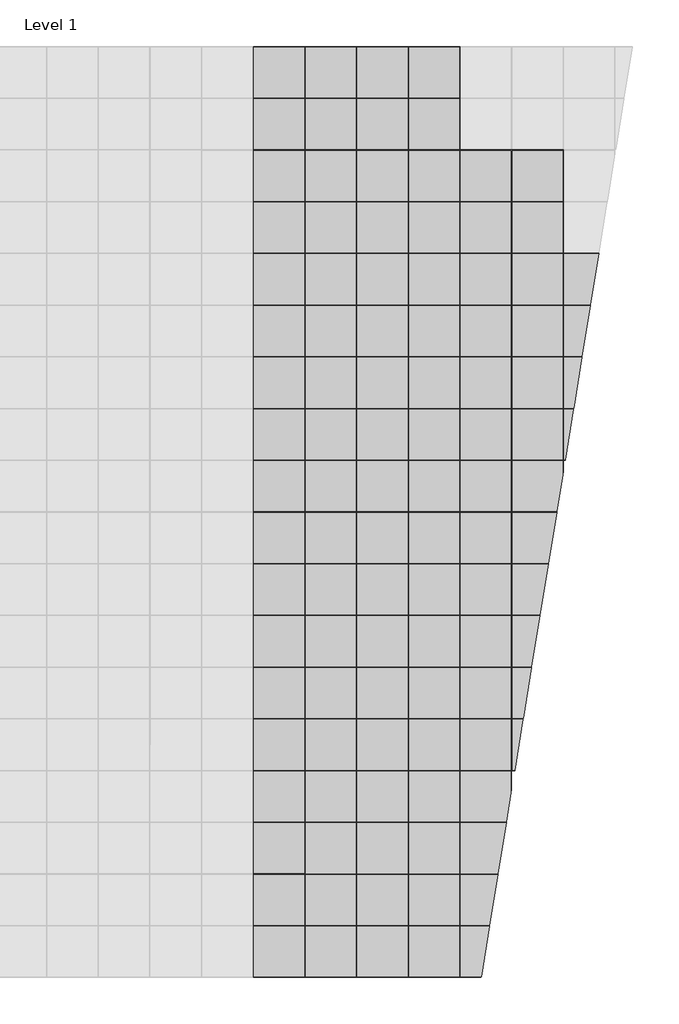
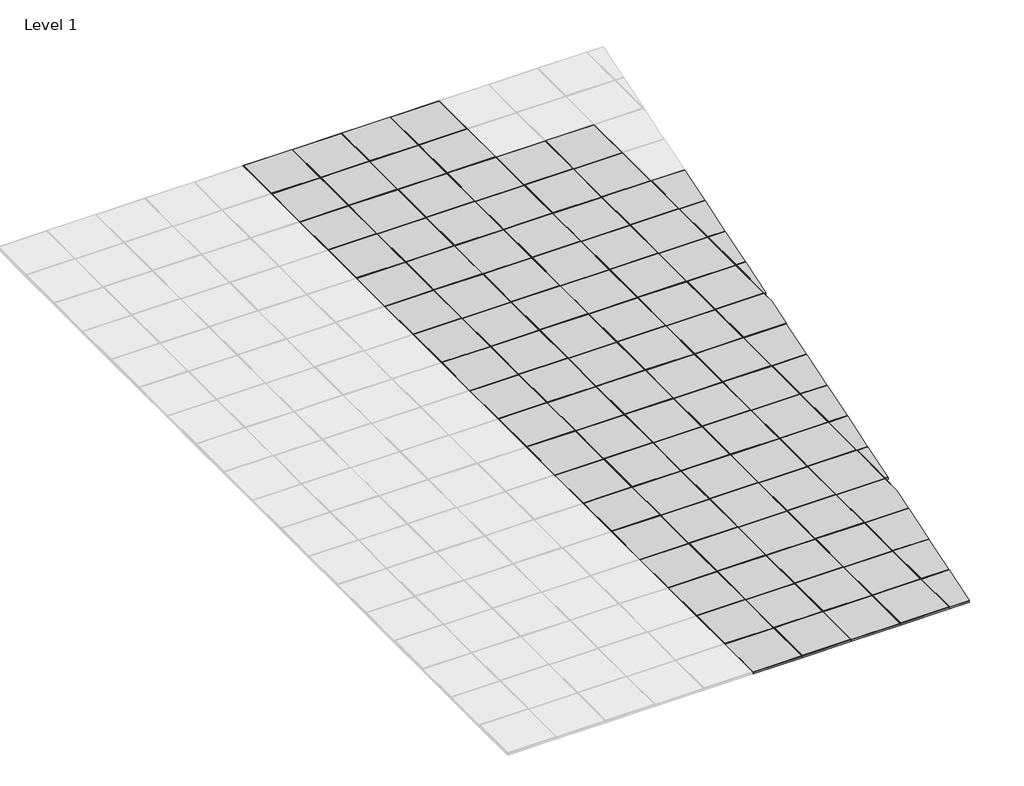
# One storey, part 2 of 18: 104 plates.
"""IFC4 building model written with IfcOpenShell, lengths in millimetres."""

import ifcopenshell
import ifcopenshell.guid

model = None  # the IFC model being written
_history = None  # IfcOwnerHistory: only IFC2X3 demands one
_inside = {}  # id of a spatial element -> (the spatial element, [elements in it])
_under = {}  # id of a project, library or spatial element -> (it, [spatial elements below it])
_declared = {}  # id of a project -> (the project, [libraries it declares])
_typed = {}  # id of a type object -> (the type object, [elements of that type])
_made_of = {}  # id of a material, layer set ... -> (it, [elements and type objects made of it])


def new_model(schema):
    """Start an empty IFC model of exactly this schema.

    Asked for "IFC4X3", IfcOpenShell would pick the latest addendum, in which some entities
    have other attributes; the version numbers below select the first issue.
    IFC2X3 requires an IfcOwnerHistory on every rooted entity: one is made here for all.
    """
    global model, _history
    if schema == "IFC4X3":
        model = ifcopenshell.file(schema_version=(4, 3, 0, 0))
    else:
        model = ifcopenshell.file(schema=schema)
    _inside.clear()
    _under.clear()
    _declared.clear()
    _typed.clear()
    _made_of.clear()
    _history = None
    if model.schema == "IFC2X3":
        org = make("IfcOrganization", Name="unknown")
        user = make(
            "IfcPersonAndOrganization",
            ThePerson=make("IfcPerson", FamilyName="unknown"),
            TheOrganization=org,
        )
        app = make(
            "IfcApplication",
            ApplicationDeveloper=org,
            Version="unknown",
            ApplicationFullName="unknown",
            ApplicationIdentifier="unknown",
        )
        _history = make(
            "IfcOwnerHistory",
            OwningUser=user,
            OwningApplication=app,
            ChangeAction="ADDED",
            CreationDate=0,
        )
    return model


def make(cls, **values):
    """One entity of the class cls with the attributes given. An attribute that is None is left unset."""
    return model.create_entity(
        cls, **{name: value for name, value in values.items() if value is not None}
    )


def rooted(cls, **values):
    """An entity with a GlobalId (a new one), such as an element, a storey or a relation."""
    return make(cls, GlobalId=ifcopenshell.guid.new(), OwnerHistory=_history, **values)


def si_unit(unit_type, name, prefix=None):
    """IfcSIUnit, for example si_unit("LENGTHUNIT", "METRE", prefix="MILLI")."""
    return make("IfcSIUnit", UnitType=unit_type, Prefix=prefix, Name=name)


def assignment(units):
    """IfcUnitAssignment: the units of a project."""
    return None if units is None else make("IfcUnitAssignment", Units=units)


def point(xyz):
    """IfcCartesianPoint."""
    return None if xyz is None else make("IfcCartesianPoint", Coordinates=xyz)


def direction(xyz):
    """IfcDirection."""
    return None if xyz is None else make("IfcDirection", DirectionRatios=xyz)


def frame(location, z_axis=None, x_axis=None):
    """IfcAxis2Placement3D, a coordinate frame: its origin and axes. An axis left out is left unset."""
    return make(
        "IfcAxis2Placement3D",
        Location=point(location),
        Axis=direction(z_axis),
        RefDirection=direction(x_axis),
    )


def origin():
    """The frame at (0, 0, 0) with its axes left unset."""
    return frame((0.0, 0.0, 0.0))


def origin_with_axes():
    """The frame at (0, 0, 0) with the z axis (0, 0, 1) and the x axis (1, 0, 0) written out."""
    return frame((0.0, 0.0, 0.0), z_axis=(0.0, 0.0, 1.0), x_axis=(1.0, 0.0, 0.0))


def place(relative_to, where):
    """IfcLocalPlacement: puts the frame where relative to a parent placement (None: the world)."""
    return make(
        "IfcLocalPlacement", PlacementRelTo=relative_to, RelativePlacement=where
    )


def context(
    kind, dimensions, precision=None, world=None, true_north=None, identifier=None
):
    """IfcGeometricRepresentationContext, for example the 3D "Model" context."""
    return make(
        "IfcGeometricRepresentationContext",
        ContextIdentifier=identifier,
        ContextType=kind,
        CoordinateSpaceDimension=dimensions,
        Precision=precision,
        WorldCoordinateSystem=world,
        TrueNorth=true_north,
    )


def project(units=None, contexts=None):
    """IfcProject with its units and contexts."""
    return rooted(
        "IfcProject",
        Name="project",
        RepresentationContexts=contexts,
        UnitsInContext=assignment(units),
    )


def spatial(cls, under=None, at=None, **own):
    """A site, building, storey or space (cls), placed at a placement, below another one or the project."""
    s = rooted(cls, ObjectPlacement=at, **own)
    if under is not None:
        _under.setdefault(under.id(), (under, []))[1].append(s)
    return s


def polyline(points):
    """IfcPolyline through the points."""
    return make("IfcPolyline", Points=[point(p) for p in points])


def outline(outer, holes=None, kind="AREA"):
    """IfcArbitraryClosedProfileDef: a profile drawn as a closed curve; with holes, ...WithVoids."""
    if holes is None:
        return make("IfcArbitraryClosedProfileDef", ProfileType=kind, OuterCurve=outer)
    return make(
        "IfcArbitraryProfileDefWithVoids",
        ProfileType=kind,
        OuterCurve=outer,
        InnerCurves=holes,
    )


def extrude(swept, where, along, depth):
    """IfcExtrudedAreaSolid: the profile swept, set in the frame where, extruded along a direction by depth."""
    return make(
        "IfcExtrudedAreaSolid",
        SweptArea=swept,
        Position=where,
        ExtrudedDirection=direction(along),
        Depth=depth,
    )


def shape(context_of_items, identifier, shape_type, items):
    """IfcShapeRepresentation: the items that make up one representation, for example the "Body"."""
    return make(
        "IfcShapeRepresentation",
        ContextOfItems=context_of_items,
        RepresentationIdentifier=identifier,
        RepresentationType=shape_type,
        Items=items,
    )


def source(mapping_origin, context_of_items, identifier, shape_type, items):
    """IfcRepresentationMap: a shape defined once, which mapped items show again and again."""
    return make(
        "IfcRepresentationMap",
        MappingOrigin=mapping_origin,
        MappedRepresentation=shape(context_of_items, identifier, shape_type, items),
    )


def transform(
    local_origin,
    x_axis=None,
    y_axis=None,
    z_axis=None,
    scale=None,
    scale2=None,
    scale3=None,
    uniform=True,
):
    """IfcCartesianTransformationOperator3D, or its non-uniform kind. x_axis, y_axis, z_axis: its Axis1, 2, 3."""
    if uniform:
        return make(
            "IfcCartesianTransformationOperator3D",
            Axis1=direction(x_axis),
            Axis2=direction(y_axis),
            LocalOrigin=point(local_origin),
            Scale=scale,
            Axis3=direction(z_axis),
        )
    return make(
        "IfcCartesianTransformationOperator3DnonUniform",
        Axis1=direction(x_axis),
        Axis2=direction(y_axis),
        LocalOrigin=point(local_origin),
        Scale=scale,
        Axis3=direction(z_axis),
        Scale2=scale2,
        Scale3=scale3,
    )


def mapped(mapping_source, mapping_target):
    """IfcMappedItem: shows the shape of a source again, moved by a transform."""
    return make(
        "IfcMappedItem", MappingSource=mapping_source, MappingTarget=mapping_target
    )


def made_of(thing, what):
    """Note that an element or type object is made of a material, layer set ...; save() writes the relation."""
    if what is not None:
        _made_of.setdefault(what.id(), (what, []))[1].append(thing)
    return thing


def element(
    cls,
    number,
    at=None,
    inside=None,
    cuts=None,
    type_object=None,
    material=None,
    context=None,
    identifier="Body",
    shape_type=None,
    held_by="IfcProductDefinitionShape",
    body=None,
    shapes=None,
    **own,
):
    """One element of the class cls, such as IfcWall. Its Tag is "e" and its number.

    at: its placement. inside: the storey or other place that contains it. cuts: it is an
    opening in that element (IfcRelVoidsElement). A single representation is given by context,
    identifier, shape_type and body (its items); several are given by shapes. held_by: the class
    of the entity that holds the representations. save() writes the other relations.
    """
    e = rooted(cls, Tag="e%d" % number, ObjectPlacement=at, **own)
    if body is not None:
        shapes = [shape(context, identifier, shape_type, body)]
    if shapes is not None:
        e.Representation = make(held_by, Representations=shapes)
    if inside is not None:
        _inside.setdefault(inside.id(), (inside, []))[1].append(e)
    if cuts is not None:
        rooted(
            "IfcRelVoidsElement", RelatingBuildingElement=cuts, RelatedOpeningElement=e
        )
    if type_object is not None:
        _typed.setdefault(type_object.id(), (type_object, []))[1].append(e)
    return made_of(e, material)


def aggregate(whole, parts):
    """IfcRelAggregates: a whole, such as a stair, and the parts it consists of."""
    return rooted("IfcRelAggregates", RelatingObject=whole, RelatedObjects=parts)


def save(model, path):
    """Write the relations noted so far, then the file.

    IfcRelAggregates (storeys below a building ...), IfcRelContainedInSpatialStructure (elements
    in a storey), IfcRelDefinesByType, IfcRelAssociatesMaterial and IfcRelDeclares: one each for
    every whole, place, type object, material and project.
    """
    for whole, parts in _under.values():
        aggregate(whole, parts)
    for where, things in _inside.values():
        rooted(
            "IfcRelContainedInSpatialStructure",
            RelatedElements=things,
            RelatingStructure=where,
        )
    for kind, things in _typed.values():
        rooted("IfcRelDefinesByType", RelatedObjects=things, RelatingType=kind)
    for what, things in _made_of.values():
        rooted("IfcRelAssociatesMaterial", RelatedObjects=things, RelatingMaterial=what)
    for by, libraries in _declared.values():
        rooted("IfcRelDeclares", RelatingContext=by, RelatedDefinitions=libraries)
    model.write(path)


def type_1_8eb2385c(model_context):
    return source(origin(), model_context, "Body", "SweptSolid", [
        extrude(outline(polyline([(1000.0, 500.0), (500.0, 500.0), (500.0, 1000.0), (1000.0, 1000.0), (1000.0, 500.0)]), holes=[polyline([(995.0, 995.0), (505.0, 995.0), (505.0, 505.0), (995.0, 505.0), (995.0, 995.0)])]), origin_with_axes(), (0.0, 0.0, 1.0), 18.0),
        extrude(outline(polyline([(505.0, 995.0), (995.0, 995.0), (995.0, 505.0), (505.0, 505.0), (505.0, 995.0)])), origin_with_axes(), (0.0, 0.0, 1.0), 20.0),
    ])


model = new_model("IFC4")

# Units and contexts
model_context = context("Model", 3, world=origin())
ifc_project = project(units=[si_unit("LENGTHUNIT", "METRE", prefix="MILLI")], contexts=[model_context])

# Site, building, storey
site = spatial("IfcSite", under=ifc_project)
building = spatial("IfcBuilding", under=site)
storey = spatial("IfcBuildingStorey", under=building, Name="Level 1", Elevation=0.0)

# Plates
placement = place(None, origin())
element("IfcPlate", 1, ObjectType="00_CPA_tegel : Type 1", at=placement, inside=storey, context=model_context, shape_type="SweptSolid", body=[
    extrude(outline(polyline([(2554.2097958, -16904.4539394), (2554.2195786, -16414.4539395), (2834.3103439, -16414.4595315), (2754.6354735, -16904.4579409), (2554.2097958, -16904.4539394)])), frame((0.0, 0.0, 1000.0), z_axis=(0.0, 0.0, 1.0), x_axis=(1.0, 0.0, 0.0)), (0.0, 0.0, 1.0), 20.0),
    extrude(outline(polyline([(2549.209696, -16909.4538396), (2549.2196784, -16409.4538397), (2835.1233527, -16409.4595477), (2834.3103439, -16414.4595315), (2554.2195786, -16414.4539395), (2554.2097958, -16904.4539394), (2754.6354735, -16904.4579409), (2753.8224647, -16909.4579246), (2549.209696, -16909.4538396)])), frame((0.0, 0.0, 1000.0), z_axis=(0.0, 0.0, 1.0), x_axis=(1.0, 0.0, 0.0)), (0.0, 0.0, 1.0), 18.0),
])
element("IfcPlate", 2, ObjectType="00_CPA_tegel : Type 1", at=placement, inside=storey, context=model_context, shape_type="SweptSolid", body=[
    extrude(outline(polyline([(2554.2197783, -16404.4539395), (2554.229561, -15914.4539396), (2915.6112321, -15914.4611545), (2835.9363617, -16404.4595639), (2554.2197783, -16404.4539395)])), frame((0.0, 0.0, 1000.0), z_axis=(0.0, 0.0, 1.0), x_axis=(1.0, 0.0, 0.0)), (0.0, 0.0, 1.0), 20.0),
    extrude(outline(polyline([(2549.2196784, -16409.4538397), (2549.2296609, -15909.4538398), (2916.424241, -15909.4611708), (2915.6112321, -15914.4611545), (2554.229561, -15914.4539396), (2554.2197783, -16404.4539395), (2835.9363617, -16404.4595639), (2835.1233528, -16409.4595477), (2549.2196784, -16409.4538397)])), frame((0.0, 0.0, 1000.0), z_axis=(0.0, 0.0, 1.0), x_axis=(1.0, 0.0, 0.0)), (0.0, 0.0, 1.0), 18.0),
])
element("IfcPlate", 3, ObjectType="00_CPA_tegel : Type 1", at=placement, inside=storey, context=model_context, shape_type="SweptSolid", body=[
    extrude(outline(polyline([(2554.2297607, -15904.4539396), (2554.2395435, -15414.4539397), (2996.9121201, -15414.4627776), (2917.2372499, -15904.461187), (2554.2297607, -15904.4539396)])), frame((0.0, 0.0, 1000.0), z_axis=(0.0, 0.0, 1.0), x_axis=(1.0, 0.0, 0.0)), (0.0, 0.0, 1.0), 20.0),
    extrude(outline(polyline([(2549.2296609, -15909.4538398), (2549.2396433, -15409.4538399), (2997.7251291, -15409.4627938), (2996.9121203, -15414.4627776), (2554.2395435, -15414.4539397), (2554.2297607, -15904.4539396), (2917.2372499, -15904.461187), (2916.424241, -15909.4611708), (2549.2296609, -15909.4538398)])), frame((0.0, 0.0, 1000.0), z_axis=(0.0, 0.0, 1.0), x_axis=(1.0, 0.0, 0.0)), (0.0, 0.0, 1.0), 18.0),
])
element("IfcPlate", 4, ObjectType="00_CPA_tegel : Type 1", at=placement, inside=storey, context=model_context, shape_type="SweptSolid", body=[
    extrude(outline(polyline([(2554.2397431, -15404.4539397), (2554.2495259, -14914.4539398), (3044.2495258, -14914.4637226), (3044.2453551, -15123.3645971), (2998.538138, -15404.4628101), (2554.2397431, -15404.4539397)])), frame((0.0, 0.0, 1000.0), z_axis=(0.0, 0.0, 1.0), x_axis=(1.0, 0.0, 0.0)), (0.0, 0.0, 1.0), 20.0),
    extrude(outline(polyline([(2549.2496257, -14909.45384), (3049.2496256, -14909.4638224), (3049.2459691, -15092.6109493), (3044.2453551, -15123.3645971), (3044.2495258, -14914.4637226), (2554.2495259, -14914.4539398), (2554.2397431, -15404.4539397), (2998.538138, -15404.4628101), (2997.7251291, -15409.4627938), (2549.2396433, -15409.4538399), (2549.2496257, -14909.45384)])), frame((0.0, 0.0, 1000.0), z_axis=(0.0, 0.0, 1.0), x_axis=(1.0, 0.0, 0.0)), (0.0, 0.0, 1.0), 18.0),
])
element("IfcPlate", 5, ObjectType="00_CPA_tegel : Type 1", at=placement, inside=storey, context=model_context, shape_type="SweptSolid", body=[
    extrude(outline(polyline([(2554.2497256, -14904.4539398), (2554.2595083, -14414.4539399), (3044.2595082, -14414.4637227), (3044.2497255, -14904.4637226), (2554.2497256, -14904.4539398)])), frame((0.0, 0.0, 1000.0), z_axis=(0.0, 0.0, 1.0), x_axis=(1.0, 0.0, 0.0)), (0.0, 0.0, 1.0), 20.0),
    extrude(outline(polyline([(3049.2496256, -14909.4638224), (2549.2496257, -14909.45384), (2549.2596082, -14409.4538401), (3049.2596081, -14409.4638225), (3049.2496256, -14909.4638224)]), holes=[polyline([(3044.2595082, -14414.4637227), (2554.2595083, -14414.4539399), (2554.2497256, -14904.4539398), (3044.2497255, -14904.4637226), (3044.2595082, -14414.4637227)])]), frame((0.0, 0.0, 1000.0), z_axis=(0.0, 0.0, 1.0), x_axis=(1.0, 0.0, 0.0)), (0.0, 0.0, 1.0), 18.0),
])
element("IfcPlate", 6, ObjectType="00_CPA_tegel : Type 1", at=placement, inside=storey, context=model_context, shape_type="SweptSolid", body=[
    extrude(outline(polyline([(3054.2497255, -14904.4639222), (3054.2595082, -14414.4639223), (3159.5138967, -14414.4660237), (3079.8390262, -14904.4644331), (3054.2497255, -14904.4639222)])), frame((0.0, 0.0, 1000.0), z_axis=(0.0, 0.0, 1.0), x_axis=(1.0, 0.0, 0.0)), (0.0, 0.0, 1.0), 20.0),
    extrude(outline(polyline([(3049.2496256, -14909.4638224), (3049.2596081, -14409.4638225), (3160.3269056, -14409.46604), (3159.5138966, -14414.4660237), (3054.2595082, -14414.4639223), (3054.2497255, -14904.4639222), (3079.8390262, -14904.4644331), (3079.0260173, -14909.4644169), (3049.2496256, -14909.4638224)])), frame((0.0, 0.0, 1000.0), z_axis=(0.0, 0.0, 1.0), x_axis=(1.0, 0.0, 0.0)), (0.0, 0.0, 1.0), 18.0),
])
element("IfcPlate", 7, ObjectType="00_CPA_tegel : Type 1", at=placement, inside=storey, context=model_context, shape_type="SweptSolid", body=[
    extrude(outline(polyline([(3554.3295848, -10904.4739055), (3554.3393676, -10414.4739056), (3809.9210017, -10414.4790082), (3730.2461314, -10904.4774176), (3554.3295848, -10904.4739055)])), frame((0.0, 0.0, 1000.0), z_axis=(0.0, 0.0, 1.0), x_axis=(1.0, 0.0, 0.0)), (0.0, 0.0, 1.0), 20.0),
    extrude(outline(polyline([(3549.329485, -10909.4738056), (3549.3394674, -10409.4738057), (3810.7340106, -10409.4790245), (3809.9210018, -10414.4790082), (3554.3393676, -10414.4739056), (3554.3295848, -10904.4739055), (3730.2461314, -10904.4774176), (3729.4331225, -10909.4774014), (3549.329485, -10909.4738056)])), frame((0.0, 0.0, 1000.0), z_axis=(0.0, 0.0, 1.0), x_axis=(1.0, 0.0, 0.0)), (0.0, 0.0, 1.0), 18.0),
])
element("IfcPlate", 8, ObjectType="00_CPA_tegel : Type 1", at=placement, inside=storey, context=model_context, shape_type="SweptSolid", body=[
    extrude(outline(polyline([(3554.3395673, -10404.4739056), (3554.34935, -9914.4739057), (3891.2218899, -9914.4806313), (3811.5470196, -10404.4790407), (3554.3395673, -10404.4739056)])), frame((0.0, 0.0, 1000.0), z_axis=(0.0, 0.0, 1.0), x_axis=(1.0, 0.0, 0.0)), (0.0, 0.0, 1.0), 20.0),
    extrude(outline(polyline([(3549.3394674, -10409.4738057), (3549.3494499, -9909.4738058), (3892.0348988, -9909.4806475), (3891.22189, -9914.4806313), (3554.34935, -9914.4739057), (3554.3395673, -10404.4739056), (3811.5470196, -10404.4790407), (3810.7340107, -10409.4790245), (3549.3394674, -10409.4738057)])), frame((0.0, 0.0, 1000.0), z_axis=(0.0, 0.0, 1.0), x_axis=(1.0, 0.0, 0.0)), (0.0, 0.0, 1.0), 18.0),
])
element("IfcPlate", 9, ObjectType="00_CPA_tegel : Type 1", at=placement, inside=storey, context=model_context, shape_type="SweptSolid", body=[
    extrude(outline(polyline([(3054.2597079, -14404.4639223), (3054.2694907, -13914.4639224), (3240.8147847, -13914.4676468), (3161.1399143, -14404.4660562), (3054.2597079, -14404.4639223)])), frame((0.0, 0.0, 1000.0), z_axis=(0.0, 0.0, 1.0), x_axis=(1.0, 0.0, 0.0)), (0.0, 0.0, 1.0), 20.0),
    extrude(outline(polyline([(3049.2596081, -14409.4638225), (3049.2695905, -13909.4638226), (3241.6277936, -13909.467663), (3240.8147847, -13914.4676468), (3054.2694907, -13914.4639224), (3054.2597079, -14404.4639223), (3161.1399143, -14404.4660562), (3160.3269054, -14409.46604), (3049.2596081, -14409.4638225)])), frame((0.0, 0.0, 1000.0), z_axis=(0.0, 0.0, 1.0), x_axis=(1.0, 0.0, 0.0)), (0.0, 0.0, 1.0), 18.0),
])
element("IfcPlate", 10, ObjectType="00_CPA_tegel : Type 1", at=placement, inside=storey, context=model_context, shape_type="SweptSolid", body=[
    extrude(outline(polyline([(3054.2696903, -13904.4639224), (3054.2794731, -13414.4639225), (3322.1156728, -13414.4692699), (3242.4408025, -13904.4676793), (3054.2696903, -13904.4639224)])), frame((0.0, 0.0, 1000.0), z_axis=(0.0, 0.0, 1.0), x_axis=(1.0, 0.0, 0.0)), (0.0, 0.0, 1.0), 20.0),
    extrude(outline(polyline([(3049.2695905, -13909.4638226), (3049.2795729, -13409.4638227), (3322.9286817, -13409.4692861), (3322.1156729, -13414.4692699), (3054.2794731, -13414.4639225), (3054.2696903, -13904.4639224), (3242.4408025, -13904.4676793), (3241.6277936, -13909.467663), (3049.2695905, -13909.4638226)])), frame((0.0, 0.0, 1000.0), z_axis=(0.0, 0.0, 1.0), x_axis=(1.0, 0.0, 0.0)), (0.0, 0.0, 1.0), 18.0),
])
element("IfcPlate", 11, ObjectType="00_CPA_tegel : Type 1", at=placement, inside=storey, context=model_context, shape_type="SweptSolid", body=[
    extrude(outline(polyline([(3054.2796728, -13404.4639225), (3054.2894555, -12914.4639226), (3403.416561, -12914.4708929), (3323.7416906, -13404.4693023), (3054.2796728, -13404.4639225)])), frame((0.0, 0.0, 1000.0), z_axis=(0.0, 0.0, 1.0), x_axis=(1.0, 0.0, 0.0)), (0.0, 0.0, 1.0), 20.0),
    extrude(outline(polyline([(3049.2795729, -13409.4638227), (3049.2895554, -12909.4638228), (3404.2295699, -12909.4709091), (3403.416561, -12914.4708929), (3054.2894555, -12914.4639226), (3054.2796728, -13404.4639225), (3323.7416906, -13404.4693023), (3322.9286818, -13409.4692861), (3049.2795729, -13409.4638227)])), frame((0.0, 0.0, 1000.0), z_axis=(0.0, 0.0, 1.0), x_axis=(1.0, 0.0, 0.0)), (0.0, 0.0, 1.0), 18.0),
])
element("IfcPlate", 12, ObjectType="00_CPA_tegel : Type 1", at=placement, inside=storey, context=model_context, shape_type="SweptSolid", body=[
    extrude(outline(polyline([(3054.2896552, -12904.4639226), (3054.299438, -12414.4639227), (3484.7174491, -12414.472516), (3405.0425788, -12904.4709254), (3054.2896552, -12904.4639226)])), frame((0.0, 0.0, 1000.0), z_axis=(0.0, 0.0, 1.0), x_axis=(1.0, 0.0, 0.0)), (0.0, 0.0, 1.0), 20.0),
    extrude(outline(polyline([(3049.2895554, -12909.4638228), (3049.2995378, -12409.4638229), (3485.5304581, -12409.4725322), (3484.7174492, -12414.472516), (3054.299438, -12414.4639227), (3054.2896552, -12904.4639226), (3405.0425788, -12904.4709254), (3404.2295699, -12909.4709091), (3049.2895554, -12909.4638228)])), frame((0.0, 0.0, 1000.0), z_axis=(0.0, 0.0, 1.0), x_axis=(1.0, 0.0, 0.0)), (0.0, 0.0, 1.0), 18.0),
])
element("IfcPlate", 13, ObjectType="00_CPA_tegel : Type 1", at=placement, inside=storey, context=model_context, shape_type="SweptSolid", body=[
    extrude(outline(polyline([(3054.2996376, -12404.4639227), (3054.3094204, -11914.4639228), (3544.3094203, -11914.4737056), (3544.3067545, -12047.9998168), (3486.343467, -12404.4725484), (3054.2996376, -12404.4639227)])), frame((0.0, 0.0, 1000.0), z_axis=(0.0, 0.0, 1.0), x_axis=(1.0, 0.0, 0.0)), (0.0, 0.0, 1.0), 20.0),
    extrude(outline(polyline([(3049.3095202, -11909.463823), (3549.3095201, -11909.4738054), (3549.3073685, -12017.246169), (3544.3067545, -12047.9998168), (3544.3094203, -11914.4737056), (3054.3094204, -11914.4639228), (3054.2996376, -12404.4639227), (3486.343467, -12404.4725484), (3485.5304581, -12409.4725322), (3049.2995378, -12409.4638229), (3049.3095202, -11909.463823)])), frame((0.0, 0.0, 1000.0), z_axis=(0.0, 0.0, 1.0), x_axis=(1.0, 0.0, 0.0)), (0.0, 0.0, 1.0), 18.0),
])
element("IfcPlate", 14, ObjectType="00_CPA_tegel : Type 1", at=placement, inside=storey, context=model_context, shape_type="SweptSolid", body=[
    extrude(outline(polyline([(3054.3096201, -11904.4639228), (3054.3194028, -11414.4639229), (3544.3194027, -11414.4737057), (3544.30962, -11904.4737056), (3054.3096201, -11904.4639228)])), frame((0.0, 0.0, 1000.0), z_axis=(0.0, 0.0, 1.0), x_axis=(1.0, 0.0, 0.0)), (0.0, 0.0, 1.0), 20.0),
    extrude(outline(polyline([(3549.3095201, -11909.4738054), (3049.3095202, -11909.463823), (3049.3195027, -11409.4638231), (3549.3195026, -11409.4738055), (3549.3095201, -11909.4738054)]), holes=[polyline([(3544.3194027, -11414.4737057), (3054.3194028, -11414.4639229), (3054.3096201, -11904.4639228), (3544.30962, -11904.4737056), (3544.3194027, -11414.4737057)])]), frame((0.0, 0.0, 1000.0), z_axis=(0.0, 0.0, 1.0), x_axis=(1.0, 0.0, 0.0)), (0.0, 0.0, 1.0), 18.0),
])
element("IfcPlate", 15, ObjectType="00_CPA_tegel : Type 1", at=placement, inside=storey, context=model_context, shape_type="SweptSolid", body=[
    extrude(outline(polyline([(3554.30962, -11904.4739053), (3554.3194027, -11414.4739054), (3647.3192254, -11414.4757621), (3567.6443551, -11904.4741715), (3554.30962, -11904.4739053)])), frame((0.0, 0.0, 1000.0), z_axis=(0.0, 0.0, 1.0), x_axis=(1.0, 0.0, 0.0)), (0.0, 0.0, 1.0), 20.0),
    extrude(outline(polyline([(3549.3095201, -11909.4738054), (3549.3195026, -11409.4738055), (3648.1322344, -11409.4757783), (3647.3192255, -11414.4757621), (3554.3194027, -11414.4739054), (3554.30962, -11904.4739053), (3567.6443551, -11904.4741715), (3566.8313462, -11909.4741553), (3549.3095201, -11909.4738054)])), frame((0.0, 0.0, 1000.0), z_axis=(0.0, 0.0, 1.0), x_axis=(1.0, 0.0, 0.0)), (0.0, 0.0, 1.0), 18.0),
])
element("IfcPlate", 16, ObjectType="00_CPA_tegel : Type 1", at=placement, inside=storey, context=model_context, shape_type="SweptSolid", body=[
    extrude(outline(polyline([(3554.3196024, -11404.4739054), (3554.3293852, -10914.4739055), (3728.6201137, -10914.4773852), (3648.9452433, -11404.4757946), (3554.3196024, -11404.4739054)])), frame((0.0, 0.0, 1000.0), z_axis=(0.0, 0.0, 1.0), x_axis=(1.0, 0.0, 0.0)), (0.0, 0.0, 1.0), 20.0),
    extrude(outline(polyline([(3549.3195026, -11409.4738055), (3549.329485, -10909.4738056), (3729.4331225, -10909.4774014), (3728.6201137, -10914.4773852), (3554.3293852, -10914.4739055), (3554.3196024, -11404.4739054), (3648.9452433, -11404.4757946), (3648.1322344, -11409.4757783), (3549.3195026, -11409.4738055)])), frame((0.0, 0.0, 1000.0), z_axis=(0.0, 0.0, 1.0), x_axis=(1.0, 0.0, 0.0)), (0.0, 0.0, 1.0), 18.0),
])
type_1_shape = type_1_8eb2385c(model_context)
element("IfcPlate", 17, ObjectType="00_CPA_tegel : Type 1", at=placement, inside=storey, context=model_context, shape_type="MappedRepresentation", body=[
    mapped(type_1_shape, transform((49.1997141, -17409.4039273, 1000.0), x_axis=(0.9999999998007024, -1.9964866676991377e-05, 0.0), y_axis=(1.9964866676991377e-05, 0.9999999998007024, 0.0), z_axis=(0.0, 0.0, 1.0))),
])
element("IfcPlate", 18, ObjectType="00_CPA_tegel : Type 1", at=placement, inside=storey, context=model_context, shape_type="MappedRepresentation", body=[
    mapped(type_1_shape, transform((549.199714, -17409.4139098, 1000.0), x_axis=(0.9999999998007022, -1.9964866676547288e-05, 0.0), y_axis=(1.9964866676547288e-05, 0.9999999998007022, 0.0), z_axis=(0.0, 0.0, 1.0))),
])
element("IfcPlate", 19, ObjectType="00_CPA_tegel : Type 1", at=placement, inside=storey, context=model_context, shape_type="MappedRepresentation", body=[
    mapped(type_1_shape, transform((49.2096965, -16909.4039274, 1000.0), x_axis=(0.9999999998007024, -1.9964866676325244e-05, 0.0), y_axis=(1.9964866676325244e-05, 0.9999999998007024, 0.0), z_axis=(0.0, 0.0, 1.0))),
])
element("IfcPlate", 20, ObjectType="00_CPA_tegel : Type 1", at=placement, inside=storey, context=model_context, shape_type="MappedRepresentation", body=[
    mapped(type_1_shape, transform((549.2096964, -16909.4139098, 1000.0), x_axis=(0.9999999998007023, -1.9964866675492576e-05, 0.0), y_axis=(1.9964866675492576e-05, 0.9999999998007023, 0.0), z_axis=(0.0, 0.0, 1.0))),
])
element("IfcPlate", 21, ObjectType="00_CPA_tegel : Type 1", at=placement, inside=storey, context=model_context, shape_type="MappedRepresentation", body=[
    mapped(type_1_shape, transform((49.2196789, -16409.4039275, 1000.0), x_axis=(0.9999999998007023, -1.9964866675492576e-05, 0.0), y_axis=(1.9964866675492576e-05, 0.9999999998007023, 0.0), z_axis=(0.0, 0.0, 1.0))),
])
element("IfcPlate", 22, ObjectType="00_CPA_tegel : Type 1", at=placement, inside=storey, context=model_context, shape_type="MappedRepresentation", body=[
    mapped(type_1_shape, transform((549.2196788, -16409.4139099, 1000.0), x_axis=(0.9999999998007023, -1.9964866675492576e-05, 0.0), y_axis=(1.9964866675492576e-05, 0.9999999998007023, 0.0), z_axis=(0.0, 0.0, 1.0))),
])
element("IfcPlate", 23, ObjectType="00_CPA_tegel : Type 1", at=placement, inside=storey, context=model_context, shape_type="MappedRepresentation", body=[
    mapped(type_1_shape, transform((49.2296614, -15909.4039276, 1000.0), x_axis=(0.9999999998007024, -1.9964866676991377e-05, 0.0), y_axis=(1.9964866676991377e-05, 0.9999999998007024, 0.0), z_axis=(0.0, 0.0, 1.0))),
])
element("IfcPlate", 24, ObjectType="00_CPA_tegel : Type 1", at=placement, inside=storey, context=model_context, shape_type="MappedRepresentation", body=[
    mapped(type_1_shape, transform((549.2296613, -15909.41391, 1000.0), x_axis=(0.9999999998007024, -1.9964866676991377e-05, 0.0), y_axis=(1.9964866676991377e-05, 0.9999999998007024, 0.0), z_axis=(0.0, 0.0, 1.0))),
])
element("IfcPlate", 25, ObjectType="00_CPA_tegel : Type 1", at=placement, inside=storey, context=model_context, shape_type="MappedRepresentation", body=[
    mapped(type_1_shape, transform((49.2396438, -15409.4039277, 1000.0), x_axis=(0.9999999998007023, -1.9964866675492576e-05, 0.0), y_axis=(1.9964866675492576e-05, 0.9999999998007023, 0.0), z_axis=(0.0, 0.0, 1.0))),
])
element("IfcPlate", 26, ObjectType="00_CPA_tegel : Type 1", at=placement, inside=storey, context=model_context, shape_type="MappedRepresentation", body=[
    mapped(type_1_shape, transform((549.2396437, -15409.4139101, 1000.0), x_axis=(0.9999999998007024, -1.9964866676991377e-05, 0.0), y_axis=(1.9964866676991377e-05, 0.9999999998007024, 0.0), z_axis=(0.0, 0.0, 1.0))),
])
element("IfcPlate", 27, ObjectType="00_CPA_tegel : Type 1", at=placement, inside=storey, context=model_context, shape_type="MappedRepresentation", body=[
    mapped(type_1_shape, transform((49.2496262, -14909.4039278, 1000.0), x_axis=(0.9999999998007024, -1.9964866676991377e-05, 0.0), y_axis=(1.9964866676991377e-05, 0.9999999998007024, 0.0), z_axis=(0.0, 0.0, 1.0))),
])
element("IfcPlate", 28, ObjectType="00_CPA_tegel : Type 1", at=placement, inside=storey, context=model_context, shape_type="MappedRepresentation", body=[
    mapped(type_1_shape, transform((549.2496261, -14909.4139102, 1000.0), x_axis=(0.9999999998007024, -1.9964866676991377e-05, 0.0), y_axis=(1.9964866676991377e-05, 0.9999999998007024, 0.0), z_axis=(0.0, 0.0, 1.0))),
])
element("IfcPlate", 29, ObjectType="00_CPA_tegel : Type 1", at=placement, inside=storey, context=model_context, shape_type="MappedRepresentation", body=[
    mapped(type_1_shape, transform((49.2596087, -14409.4039279, 1000.0), x_axis=(0.9999999998007024, -1.9964866676991377e-05, 0.0), y_axis=(1.9964866676991377e-05, 0.9999999998007024, 0.0), z_axis=(0.0, 0.0, 1.0))),
])
element("IfcPlate", 30, ObjectType="00_CPA_tegel : Type 1", at=placement, inside=storey, context=model_context, shape_type="MappedRepresentation", body=[
    mapped(type_1_shape, transform((549.2596086, -14409.4139103, 1000.0), x_axis=(0.9999999998007024, -1.9964866676991377e-05, 0.0), y_axis=(1.9964866676991377e-05, 0.9999999998007024, 0.0), z_axis=(0.0, 0.0, 1.0))),
])
element("IfcPlate", 31, ObjectType="00_CPA_tegel : Type 1", at=placement, inside=storey, context=model_context, shape_type="MappedRepresentation", body=[
    mapped(type_1_shape, transform((49.2695911, -13909.403928, 1000.0), x_axis=(0.9999999998007022, -1.9964866678323645e-05, 0.0), y_axis=(1.9964866678323645e-05, 0.9999999998007022, 0.0), z_axis=(0.0, 0.0, 1.0))),
])
element("IfcPlate", 32, ObjectType="00_CPA_tegel : Type 1", at=placement, inside=storey, context=model_context, shape_type="MappedRepresentation", body=[
    mapped(type_1_shape, transform((549.269591, -13909.4139104, 1000.0), x_axis=(0.9999999998007024, -1.9964866676991377e-05, 0.0), y_axis=(1.9964866676991377e-05, 0.9999999998007024, 0.0), z_axis=(0.0, 0.0, 1.0))),
])
element("IfcPlate", 33, ObjectType="00_CPA_tegel : Type 1", at=placement, inside=storey, context=model_context, shape_type="MappedRepresentation", body=[
    mapped(type_1_shape, transform((49.2795735, -13409.4039281, 1000.0), x_axis=(0.9999999998007022, -1.9964866678323645e-05, 0.0), y_axis=(1.9964866678323645e-05, 0.9999999998007022, 0.0), z_axis=(0.0, 0.0, 1.0))),
])
element("IfcPlate", 34, ObjectType="00_CPA_tegel : Type 1", at=placement, inside=storey, context=model_context, shape_type="MappedRepresentation", body=[
    mapped(type_1_shape, transform((549.2795734, -13409.4139105, 1000.0), x_axis=(0.9999999998007024, -1.9964866676991377e-05, 0.0), y_axis=(1.9964866676991377e-05, 0.9999999998007024, 0.0), z_axis=(0.0, 0.0, 1.0))),
])
element("IfcPlate", 35, ObjectType="00_CPA_tegel : Type 1", at=placement, inside=storey, context=model_context, shape_type="MappedRepresentation", body=[
    mapped(type_1_shape, transform((1049.1997139, -17409.4238922, 1000.0), x_axis=(0.9999999998007023, -1.996486667804609e-05, 0.0), y_axis=(1.996486667804609e-05, 0.9999999998007023, 0.0), z_axis=(0.0, 0.0, 1.0))),
])
element("IfcPlate", 36, ObjectType="00_CPA_tegel : Type 1", at=placement, inside=storey, context=model_context, shape_type="MappedRepresentation", body=[
    mapped(type_1_shape, transform((1049.2096963, -16909.4238923, 1000.0), x_axis=(0.9999999998007024, -1.9964866676991377e-05, 0.0), y_axis=(1.9964866676991377e-05, 0.9999999998007024, 0.0), z_axis=(0.0, 0.0, 1.0))),
])
element("IfcPlate", 37, ObjectType="00_CPA_tegel : Type 1", at=placement, inside=storey, context=model_context, shape_type="MappedRepresentation", body=[
    mapped(type_1_shape, transform((1049.2196787, -16409.4238924, 1000.0), x_axis=(0.9999999998007022, -1.9964866678323645e-05, 0.0), y_axis=(1.9964866678323645e-05, 0.9999999998007022, 0.0), z_axis=(0.0, 0.0, 1.0))),
])
element("IfcPlate", 38, ObjectType="00_CPA_tegel : Type 1", at=placement, inside=storey, context=model_context, shape_type="MappedRepresentation", body=[
    mapped(type_1_shape, transform((1549.2096962, -16909.4338747, 1000.0), x_axis=(0.9999999998007024, -1.9964866676325244e-05, 0.0), y_axis=(1.9964866676325244e-05, 0.9999999998007024, 0.0), z_axis=(0.0, 0.0, 1.0))),
])
element("IfcPlate", 39, ObjectType="00_CPA_tegel : Type 1", at=placement, inside=storey, context=model_context, shape_type="MappedRepresentation", body=[
    mapped(type_1_shape, transform((1549.2196786, -16409.4338748, 1000.0), x_axis=(0.9999999998007024, -1.9964866676991377e-05, 0.0), y_axis=(1.9964866676991377e-05, 0.9999999998007024, 0.0), z_axis=(0.0, 0.0, 1.0))),
])
element("IfcPlate", 40, ObjectType="00_CPA_tegel : Type 1", at=placement, inside=storey, context=model_context, shape_type="MappedRepresentation", body=[
    mapped(type_1_shape, transform((1049.2296612, -15909.4238925, 1000.0), x_axis=(0.9999999998007022, -1.9964866678323645e-05, 0.0), y_axis=(1.9964866678323645e-05, 0.9999999998007022, 0.0), z_axis=(0.0, 0.0, 1.0))),
])
element("IfcPlate", 41, ObjectType="00_CPA_tegel : Type 1", at=placement, inside=storey, context=model_context, shape_type="MappedRepresentation", body=[
    mapped(type_1_shape, transform((1549.2296611, -15909.4338749, 1000.0), x_axis=(0.9999999998007024, -1.9964866676991377e-05, 0.0), y_axis=(1.9964866676991377e-05, 0.9999999998007024, 0.0), z_axis=(0.0, 0.0, 1.0))),
])
element("IfcPlate", 42, ObjectType="00_CPA_tegel : Type 1", at=placement, inside=storey, context=model_context, shape_type="MappedRepresentation", body=[
    mapped(type_1_shape, transform((1049.2396436, -15409.4238926, 1000.0), x_axis=(0.9999999998007024, -1.9964866676991377e-05, 0.0), y_axis=(1.9964866676991377e-05, 0.9999999998007024, 0.0), z_axis=(0.0, 0.0, 1.0))),
])
element("IfcPlate", 43, ObjectType="00_CPA_tegel : Type 1", at=placement, inside=storey, context=model_context, shape_type="MappedRepresentation", body=[
    mapped(type_1_shape, transform((1049.249626, -14909.4238927, 1000.0), x_axis=(0.9999999998007023, -1.9964866675492576e-05, 0.0), y_axis=(1.9964866675492576e-05, 0.9999999998007023, 0.0), z_axis=(0.0, 0.0, 1.0))),
])
element("IfcPlate", 44, ObjectType="00_CPA_tegel : Type 1", at=placement, inside=storey, context=model_context, shape_type="MappedRepresentation", body=[
    mapped(type_1_shape, transform((1049.2596085, -14409.4238928, 1000.0), x_axis=(0.9999999998007022, -1.9964866678323645e-05, 0.0), y_axis=(1.9964866678323645e-05, 0.9999999998007022, 0.0), z_axis=(0.0, 0.0, 1.0))),
])
element("IfcPlate", 45, ObjectType="00_CPA_tegel : Type 1", at=placement, inside=storey, context=model_context, shape_type="MappedRepresentation", body=[
    mapped(type_1_shape, transform((1049.2695909, -13909.4238929, 1000.0), x_axis=(0.9999999998007022, -1.9964866678323645e-05, 0.0), y_axis=(1.9964866678323645e-05, 0.9999999998007022, 0.0), z_axis=(0.0, 0.0, 1.0))),
])
element("IfcPlate", 46, ObjectType="00_CPA_tegel : Type 1", at=placement, inside=storey, context=model_context, shape_type="MappedRepresentation", body=[
    mapped(type_1_shape, transform((1049.2795733, -13409.423893, 1000.0), x_axis=(0.9999999998007024, -1.9964866676991377e-05, 0.0), y_axis=(1.9964866676991377e-05, 0.9999999998007024, 0.0), z_axis=(0.0, 0.0, 1.0))),
])
element("IfcPlate", 47, ObjectType="00_CPA_tegel : Type 1", at=placement, inside=storey, context=model_context, shape_type="MappedRepresentation", body=[
    mapped(type_1_shape, transform((1549.2396435, -15409.433875, 1000.0), x_axis=(0.9999999998007024, -1.9964866676991377e-05, 0.0), y_axis=(1.9964866676991377e-05, 0.9999999998007024, 0.0), z_axis=(0.0, 0.0, 1.0))),
])
element("IfcPlate", 48, ObjectType="00_CPA_tegel : Type 1", at=placement, inside=storey, context=model_context, shape_type="MappedRepresentation", body=[
    mapped(type_1_shape, transform((1549.2496259, -14909.4338751, 1000.0), x_axis=(0.9999999998007022, -1.9964866678323645e-05, 0.0), y_axis=(1.9964866678323645e-05, 0.9999999998007022, 0.0), z_axis=(0.0, 0.0, 1.0))),
])
element("IfcPlate", 49, ObjectType="00_CPA_tegel : Type 1", at=placement, inside=storey, context=model_context, shape_type="MappedRepresentation", body=[
    mapped(type_1_shape, transform((1549.2596084, -14409.4338752, 1000.0), x_axis=(0.9999999998007024, -1.9964866676991377e-05, 0.0), y_axis=(1.9964866676991377e-05, 0.9999999998007024, 0.0), z_axis=(0.0, 0.0, 1.0))),
])
element("IfcPlate", 50, ObjectType="00_CPA_tegel : Type 1", at=placement, inside=storey, context=model_context, shape_type="MappedRepresentation", body=[
    mapped(type_1_shape, transform((1549.2695908, -13909.4338753, 1000.0), x_axis=(0.9999999998007024, -1.9964866676991377e-05, 0.0), y_axis=(1.9964866676991377e-05, 0.9999999998007024, 0.0), z_axis=(0.0, 0.0, 1.0))),
])
element("IfcPlate", 51, ObjectType="00_CPA_tegel : Type 1", at=placement, inside=storey, context=model_context, shape_type="MappedRepresentation", body=[
    mapped(type_1_shape, transform((1549.2795732, -13409.4338754, 1000.0), x_axis=(0.9999999998007022, -1.9964866678323645e-05, 0.0), y_axis=(1.9964866678323645e-05, 0.9999999998007022, 0.0), z_axis=(0.0, 0.0, 1.0))),
])
element("IfcPlate", 52, ObjectType="00_CPA_tegel : Type 1", at=placement, inside=storey, context=model_context, shape_type="MappedRepresentation", body=[
    mapped(type_1_shape, transform((49.289556, -12909.4039282, 1000.0), x_axis=(0.9999999998007023, -1.9964866675492576e-05, 0.0), y_axis=(1.9964866675492576e-05, 0.9999999998007023, 0.0), z_axis=(0.0, 0.0, 1.0))),
])
element("IfcPlate", 53, ObjectType="00_CPA_tegel : Type 1", at=placement, inside=storey, context=model_context, shape_type="MappedRepresentation", body=[
    mapped(type_1_shape, transform((549.2895559, -12909.4139106, 1000.0), x_axis=(0.9999999998007023, -1.9964866675492576e-05, 0.0), y_axis=(1.9964866675492576e-05, 0.9999999998007023, 0.0), z_axis=(0.0, 0.0, 1.0))),
])
element("IfcPlate", 54, ObjectType="00_CPA_tegel : Type 1", at=placement, inside=storey, context=model_context, shape_type="MappedRepresentation", body=[
    mapped(type_1_shape, transform((1049.2895558, -12909.4238931, 1000.0), x_axis=(0.9999999998007023, -1.9964866675492576e-05, 0.0), y_axis=(1.9964866675492576e-05, 0.9999999998007023, 0.0), z_axis=(0.0, 0.0, 1.0))),
])
element("IfcPlate", 55, ObjectType="00_CPA_tegel : Type 1", at=placement, inside=storey, context=model_context, shape_type="MappedRepresentation", body=[
    mapped(type_1_shape, transform((1549.2895557, -12909.4338755, 1000.0), x_axis=(0.9999999998007022, -1.9964866678323645e-05, 0.0), y_axis=(1.9964866678323645e-05, 0.9999999998007022, 0.0), z_axis=(0.0, 0.0, 1.0))),
])
element("IfcPlate", 56, ObjectType="00_CPA_tegel : Type 1", at=placement, inside=storey, context=model_context, shape_type="MappedRepresentation", body=[
    mapped(type_1_shape, transform((1549.2995381, -12409.4338756, 1000.0), x_axis=(0.9999999998007023, -1.9964866675492576e-05, 0.0), y_axis=(1.9964866675492576e-05, 0.9999999998007023, 0.0), z_axis=(0.0, 0.0, 1.0))),
])
element("IfcPlate", 57, ObjectType="00_CPA_tegel : Type 1", at=placement, inside=storey, context=model_context, shape_type="MappedRepresentation", body=[
    mapped(type_1_shape, transform((549.2995383, -12409.4139107, 1000.0), x_axis=(0.9999999998007022, -1.9964866678323645e-05, 0.0), y_axis=(1.9964866678323645e-05, 0.9999999998007022, 0.0), z_axis=(0.0, 0.0, 1.0))),
])
element("IfcPlate", 58, ObjectType="00_CPA_tegel : Type 1", at=placement, inside=storey, context=model_context, shape_type="MappedRepresentation", body=[
    mapped(type_1_shape, transform((1049.2995382, -12409.4238932, 1000.0), x_axis=(0.9999999998007022, -1.9964866678323645e-05, 0.0), y_axis=(1.9964866678323645e-05, 0.9999999998007022, 0.0), z_axis=(0.0, 0.0, 1.0))),
])
element("IfcPlate", 59, ObjectType="00_CPA_tegel : Type 1", at=placement, inside=storey, context=model_context, shape_type="MappedRepresentation", body=[
    mapped(type_1_shape, transform((1549.1997138, -17409.4338746, 1000.0), x_axis=(0.9999999998007024, -1.9964866676991377e-05, 0.0), y_axis=(1.9964866676991377e-05, 0.9999999998007024, 0.0), z_axis=(0.0, 0.0, 1.0))),
])
element("IfcPlate", 60, ObjectType="00_CPA_tegel : Type 1", at=placement, inside=storey, context=model_context, shape_type="MappedRepresentation", body=[
    mapped(type_1_shape, transform((49.2995384, -12409.4039283, 1000.0), x_axis=(0.9999999998007023, -1.9964866675492576e-05, 0.0), y_axis=(1.9964866675492576e-05, 0.9999999998007023, 0.0), z_axis=(0.0, 0.0, 1.0))),
])
element("IfcPlate", 61, ObjectType="00_CPA_tegel : Type 1", at=placement, inside=storey, context=model_context, shape_type="MappedRepresentation", body=[
    mapped(type_1_shape, transform((1049.3095206, -11909.4238933, 1000.0), x_axis=(0.9999999998007024, -1.9964866676991377e-05, 0.0), y_axis=(1.9964866676991377e-05, 0.9999999998007024, 0.0), z_axis=(0.0, 0.0, 1.0))),
])
element("IfcPlate", 62, ObjectType="00_CPA_tegel : Type 1", at=placement, inside=storey, context=model_context, shape_type="MappedRepresentation", body=[
    mapped(type_1_shape, transform((1549.3095205, -11909.4338757, 1000.0), x_axis=(0.9999999998007022, -1.9964866678323645e-05, 0.0), y_axis=(1.9964866678323645e-05, 0.9999999998007022, 0.0), z_axis=(0.0, 0.0, 1.0))),
])
element("IfcPlate", 63, ObjectType="00_CPA_tegel : Type 1", at=placement, inside=storey, context=model_context, shape_type="MappedRepresentation", body=[
    mapped(type_1_shape, transform((49.3195033, -11409.4039285, 1000.0), x_axis=(0.9999999998007023, -1.9964866675492576e-05, 0.0), y_axis=(1.9964866675492576e-05, 0.9999999998007023, 0.0), z_axis=(0.0, 0.0, 1.0))),
])
element("IfcPlate", 64, ObjectType="00_CPA_tegel : Type 1", at=placement, inside=storey, context=model_context, shape_type="MappedRepresentation", body=[
    mapped(type_1_shape, transform((2049.3294853, -10909.4438583, 1000.0), x_axis=(0.9999999998007022, -1.9964866678323645e-05, 0.0), y_axis=(1.9964866678323645e-05, 0.9999999998007022, 0.0), z_axis=(0.0, 0.0, 1.0))),
])
element("IfcPlate", 65, ObjectType="00_CPA_tegel : Type 1", at=placement, inside=storey, context=model_context, shape_type="MappedRepresentation", body=[
    mapped(type_1_shape, transform((2549.3294852, -10909.4538408, 1000.0), x_axis=(0.9999999998007022, -1.9964866679711424e-05, 0.0), y_axis=(1.9964866679711424e-05, 0.9999999998007022, 0.0), z_axis=(0.0, 0.0, 1.0))),
])
element("IfcPlate", 66, ObjectType="00_CPA_tegel : Type 1", at=placement, inside=storey, context=model_context, shape_type="MappedRepresentation", body=[
    mapped(type_1_shape, transform((1549.3294854, -10909.4338759, 1000.0), x_axis=(0.9999999998007022, -1.9964866678323645e-05, 0.0), y_axis=(1.9964866678323645e-05, 0.9999999998007022, 0.0), z_axis=(0.0, 0.0, 1.0))),
])
element("IfcPlate", 67, ObjectType="00_CPA_tegel : Type 1", at=placement, inside=storey, context=model_context, shape_type="MappedRepresentation", body=[
    mapped(type_1_shape, transform((2049.2496258, -14909.4438575, 1000.0), x_axis=(0.9999999998007024, -1.9964866676991377e-05, 0.0), y_axis=(1.9964866676991377e-05, 0.9999999998007024, 0.0), z_axis=(0.0, 0.0, 1.0))),
])
element("IfcPlate", 68, ObjectType="00_CPA_tegel : Type 1", at=placement, inside=storey, context=model_context, shape_type="MappedRepresentation", body=[
    mapped(type_1_shape, transform((2049.2596083, -14409.4438576, 1000.0), x_axis=(0.9999999998007024, -1.9964866676991377e-05, 0.0), y_axis=(1.9964866676991377e-05, 0.9999999998007024, 0.0), z_axis=(0.0, 0.0, 1.0))),
])
element("IfcPlate", 69, ObjectType="00_CPA_tegel : Type 1", at=placement, inside=storey, context=model_context, shape_type="MappedRepresentation", body=[
    mapped(type_1_shape, transform((2049.2695907, -13909.4438577, 1000.0), x_axis=(0.9999999998007022, -1.9964866678323645e-05, 0.0), y_axis=(1.9964866678323645e-05, 0.9999999998007022, 0.0), z_axis=(0.0, 0.0, 1.0))),
])
element("IfcPlate", 70, ObjectType="00_CPA_tegel : Type 1", at=placement, inside=storey, context=model_context, shape_type="MappedRepresentation", body=[
    mapped(type_1_shape, transform((2049.2795731, -13409.4438578, 1000.0), x_axis=(0.9999999998007024, -1.9964866676991377e-05, 0.0), y_axis=(1.9964866676991377e-05, 0.9999999998007024, 0.0), z_axis=(0.0, 0.0, 1.0))),
])
element("IfcPlate", 71, ObjectType="00_CPA_tegel : Type 1", at=placement, inside=storey, context=model_context, shape_type="MappedRepresentation", body=[
    mapped(type_1_shape, transform((2049.2895556, -12909.4438579, 1000.0), x_axis=(0.9999999998007024, -1.9964866676991377e-05, 0.0), y_axis=(1.9964866676991377e-05, 0.9999999998007024, 0.0), z_axis=(0.0, 0.0, 1.0))),
])
element("IfcPlate", 72, ObjectType="00_CPA_tegel : Type 1", at=placement, inside=storey, context=model_context, shape_type="MappedRepresentation", body=[
    mapped(type_1_shape, transform((2049.299538, -12409.443858, 1000.0), x_axis=(0.9999999998007024, -1.9964866676991377e-05, 0.0), y_axis=(1.9964866676991377e-05, 0.9999999998007024, 0.0), z_axis=(0.0, 0.0, 1.0))),
])
element("IfcPlate", 73, ObjectType="00_CPA_tegel : Type 1", at=placement, inside=storey, context=model_context, shape_type="MappedRepresentation", body=[
    mapped(type_1_shape, transform((2549.3095203, -11909.4538406, 1000.0), x_axis=(0.9999999998007022, -1.9964866679711424e-05, 0.0), y_axis=(1.9964866679711424e-05, 0.9999999998007022, 0.0), z_axis=(0.0, 0.0, 1.0))),
])
element("IfcPlate", 74, ObjectType="00_CPA_tegel : Type 1", at=placement, inside=storey, context=model_context, shape_type="MappedRepresentation", body=[
    mapped(type_1_shape, transform((2049.3095204, -11909.4438581, 1000.0), x_axis=(0.9999999998007022, -1.9964866678323645e-05, 0.0), y_axis=(1.9964866678323645e-05, 0.9999999998007022, 0.0), z_axis=(0.0, 0.0, 1.0))),
])
element("IfcPlate", 75, ObjectType="00_CPA_tegel : Type 1", at=placement, inside=storey, context=model_context, shape_type="MappedRepresentation", body=[
    mapped(type_1_shape, transform((49.3095208, -11909.4039284, 1000.0), x_axis=(0.9999999998007022, -1.9964866678323645e-05, 0.0), y_axis=(1.9964866678323645e-05, 0.9999999998007022, 0.0), z_axis=(0.0, 0.0, 1.0))),
])
element("IfcPlate", 76, ObjectType="00_CPA_tegel : Type 1", at=placement, inside=storey, context=model_context, shape_type="MappedRepresentation", body=[
    mapped(type_1_shape, transform((549.3095207, -11909.4139108, 1000.0), x_axis=(0.9999999998007022, -1.9964866678323645e-05, 0.0), y_axis=(1.9964866678323645e-05, 0.9999999998007022, 0.0), z_axis=(0.0, 0.0, 1.0))),
])
element("IfcPlate", 77, ObjectType="00_CPA_tegel : Type 1", at=placement, inside=storey, context=model_context, shape_type="MappedRepresentation", body=[
    mapped(type_1_shape, transform((549.3195032, -11409.4139109, 1000.0), x_axis=(0.9999999998007024, -1.9964866676991377e-05, 0.0), y_axis=(1.9964866676991377e-05, 0.9999999998007024, 0.0), z_axis=(0.0, 0.0, 1.0))),
])
element("IfcPlate", 78, ObjectType="00_CPA_tegel : Type 1", at=placement, inside=storey, context=model_context, shape_type="MappedRepresentation", body=[
    mapped(type_1_shape, transform((1049.3195031, -11409.4238934, 1000.0), x_axis=(0.9999999998007024, -1.9964866676991377e-05, 0.0), y_axis=(1.9964866676991377e-05, 0.9999999998007024, 0.0), z_axis=(0.0, 0.0, 1.0))),
])
element("IfcPlate", 79, ObjectType="00_CPA_tegel : Type 1", at=placement, inside=storey, context=model_context, shape_type="MappedRepresentation", body=[
    mapped(type_1_shape, transform((1549.319503, -11409.4338758, 1000.0), x_axis=(0.9999999998007024, -1.9964866676991377e-05, 0.0), y_axis=(1.9964866676991377e-05, 0.9999999998007024, 0.0), z_axis=(0.0, 0.0, 1.0))),
])
element("IfcPlate", 80, ObjectType="00_CPA_tegel : Type 1", at=placement, inside=storey, context=model_context, shape_type="MappedRepresentation", body=[
    mapped(type_1_shape, transform((2049.3195029, -11409.4438582, 1000.0), x_axis=(0.9999999998007024, -1.9964866676991377e-05, 0.0), y_axis=(1.9964866676991377e-05, 0.9999999998007024, 0.0), z_axis=(0.0, 0.0, 1.0))),
])
element("IfcPlate", 81, ObjectType="00_CPA_tegel : Type 1", at=placement, inside=storey, context=model_context, shape_type="MappedRepresentation", body=[
    mapped(type_1_shape, transform((2549.3195028, -11409.4538407, 1000.0), x_axis=(0.9999999998007024, -1.9964866676991377e-05, 0.0), y_axis=(1.9964866676991377e-05, 0.9999999998007024, 0.0), z_axis=(0.0, 0.0, 1.0))),
])
element("IfcPlate", 82, ObjectType="00_CPA_tegel : Type 1", at=placement, inside=storey, context=model_context, shape_type="MappedRepresentation", body=[
    mapped(type_1_shape, transform((49.3294857, -10909.4039286, 1000.0), x_axis=(0.9999999998007022, -1.9964866678323645e-05, 0.0), y_axis=(1.9964866678323645e-05, 0.9999999998007022, 0.0), z_axis=(0.0, 0.0, 1.0))),
])
element("IfcPlate", 83, ObjectType="00_CPA_tegel : Type 1", at=placement, inside=storey, context=model_context, shape_type="MappedRepresentation", body=[
    mapped(type_1_shape, transform((549.3294856, -10909.413911, 1000.0), x_axis=(0.9999999998007022, -1.9964866678323645e-05, 0.0), y_axis=(1.9964866678323645e-05, 0.9999999998007022, 0.0), z_axis=(0.0, 0.0, 1.0))),
])
element("IfcPlate", 84, ObjectType="00_CPA_tegel : Type 1", at=placement, inside=storey, context=model_context, shape_type="MappedRepresentation", body=[
    mapped(type_1_shape, transform((1049.3294855, -10909.4238935, 1000.0), x_axis=(0.9999999998007024, -1.9964866676991377e-05, 0.0), y_axis=(1.9964866676991377e-05, 0.9999999998007024, 0.0), z_axis=(0.0, 0.0, 1.0))),
])
element("IfcPlate", 85, ObjectType="00_CPA_tegel : Type 1", at=placement, inside=storey, context=model_context, shape_type="MappedRepresentation", body=[
    mapped(type_1_shape, transform((49.3394681, -10409.4039287, 1000.0), x_axis=(0.9999999998007022, -1.9964866678323645e-05, 0.0), y_axis=(1.9964866678323645e-05, 0.9999999998007022, 0.0), z_axis=(0.0, 0.0, 1.0))),
])
element("IfcPlate", 86, ObjectType="00_CPA_tegel : Type 1", at=placement, inside=storey, context=model_context, shape_type="MappedRepresentation", body=[
    mapped(type_1_shape, transform((549.339468, -10409.4139111, 1000.0), x_axis=(0.9999999998007022, -1.9964866678323645e-05, 0.0), y_axis=(1.9964866678323645e-05, 0.9999999998007022, 0.0), z_axis=(0.0, 0.0, 1.0))),
])
element("IfcPlate", 87, ObjectType="00_CPA_tegel : Type 1", at=placement, inside=storey, context=model_context, shape_type="MappedRepresentation", body=[
    mapped(type_1_shape, transform((1049.3394679, -10409.4238936, 1000.0), x_axis=(0.9999999998007024, -1.9964866676991377e-05, 0.0), y_axis=(1.9964866676991377e-05, 0.9999999998007024, 0.0), z_axis=(0.0, 0.0, 1.0))),
])
element("IfcPlate", 88, ObjectType="00_CPA_tegel : Type 1", at=placement, inside=storey, context=model_context, shape_type="MappedRepresentation", body=[
    mapped(type_1_shape, transform((1549.3394678, -10409.433876, 1000.0), x_axis=(0.9999999998007022, -1.9964866679711424e-05, 0.0), y_axis=(1.9964866679711424e-05, 0.9999999998007022, 0.0), z_axis=(0.0, 0.0, 1.0))),
])
element("IfcPlate", 89, ObjectType="00_CPA_tegel : Type 1", at=placement, inside=storey, context=model_context, shape_type="MappedRepresentation", body=[
    mapped(type_1_shape, transform((2049.3394677, -10409.4438584, 1000.0), x_axis=(0.9999999998007023, -1.9964866675492576e-05, 0.0), y_axis=(1.9964866675492576e-05, 0.9999999998007023, 0.0), z_axis=(0.0, 0.0, 1.0))),
])
element("IfcPlate", 90, ObjectType="00_CPA_tegel : Type 1", at=placement, inside=storey, context=model_context, shape_type="MappedRepresentation", body=[
    mapped(type_1_shape, transform((2549.3394676, -10409.4538409, 1000.0), x_axis=(0.9999999998007022, -1.9964866679711424e-05, 0.0), y_axis=(1.9964866679711424e-05, 0.9999999998007022, 0.0), z_axis=(0.0, 0.0, 1.0))),
])
element("IfcPlate", 91, ObjectType="00_CPA_tegel : Type 1", at=placement, inside=storey, context=model_context, shape_type="MappedRepresentation", body=[
    mapped(type_1_shape, transform((49.3494506, -9909.4039288, 1000.0), x_axis=(0.9999999998007023, -1.9964866675492576e-05, 0.0), y_axis=(1.9964866675492576e-05, 0.9999999998007023, 0.0), z_axis=(0.0, 0.0, 1.0))),
])
element("IfcPlate", 92, ObjectType="00_CPA_tegel : Type 1", at=placement, inside=storey, context=model_context, shape_type="MappedRepresentation", body=[
    mapped(type_1_shape, transform((549.3494505, -9909.4139112, 1000.0), x_axis=(0.9999999998007023, -1.9964866675492576e-05, 0.0), y_axis=(1.9964866675492576e-05, 0.9999999998007023, 0.0), z_axis=(0.0, 0.0, 1.0))),
])
element("IfcPlate", 93, ObjectType="00_CPA_tegel : Type 1", at=placement, inside=storey, context=model_context, shape_type="MappedRepresentation", body=[
    mapped(type_1_shape, transform((1049.3494504, -9909.4238937, 1000.0), x_axis=(0.9999999998007022, -1.9964866678323645e-05, 0.0), y_axis=(1.9964866678323645e-05, 0.9999999998007022, 0.0), z_axis=(0.0, 0.0, 1.0))),
])
element("IfcPlate", 94, ObjectType="00_CPA_tegel : Type 1", at=placement, inside=storey, context=model_context, shape_type="MappedRepresentation", body=[
    mapped(type_1_shape, transform((1549.3494503, -9909.4338761, 1000.0), x_axis=(0.9999999998007022, -1.9964866679711424e-05, 0.0), y_axis=(1.9964866679711424e-05, 0.9999999998007022, 0.0), z_axis=(0.0, 0.0, 1.0))),
])
element("IfcPlate", 95, ObjectType="00_CPA_tegel : Type 1", at=placement, inside=storey, context=model_context, shape_type="MappedRepresentation", body=[
    mapped(type_1_shape, transform((2049.3494502, -9909.4438585, 1000.0), x_axis=(0.9999999998007022, -1.9964866679711424e-05, 0.0), y_axis=(1.9964866679711424e-05, 0.9999999998007022, 0.0), z_axis=(0.0, 0.0, 1.0))),
])
element("IfcPlate", 96, ObjectType="00_CPA_tegel : Type 1", at=placement, inside=storey, context=model_context, shape_type="MappedRepresentation", body=[
    mapped(type_1_shape, transform((2549.3494501, -9909.453841, 1000.0), x_axis=(0.9999999998007022, -1.996486668248698e-05, 0.0), y_axis=(1.996486668248698e-05, 0.9999999998007022, 0.0), z_axis=(0.0, 0.0, 1.0))),
])
element("IfcPlate", 97, ObjectType="00_CPA_tegel : Type 1", at=placement, inside=storey, context=model_context, shape_type="MappedRepresentation", body=[
    mapped(type_1_shape, transform((49.359433, -9409.4039289, 1000.0), x_axis=(0.9999999998007023, -1.9964866681099203e-05, 0.0), y_axis=(1.9964866681099203e-05, 0.9999999998007023, 0.0), z_axis=(0.0, 0.0, 1.0))),
])
element("IfcPlate", 98, ObjectType="00_CPA_tegel : Type 1", at=placement, inside=storey, context=model_context, shape_type="MappedRepresentation", body=[
    mapped(type_1_shape, transform((549.3594329, -9409.4139113, 1000.0), x_axis=(0.9999999998007022, -1.996486667416031e-05, 0.0), y_axis=(1.996486667416031e-05, 0.9999999998007022, 0.0), z_axis=(0.0, 0.0, 1.0))),
])
element("IfcPlate", 99, ObjectType="00_CPA_tegel : Type 1", at=placement, inside=storey, context=model_context, shape_type="MappedRepresentation", body=[
    mapped(type_1_shape, transform((1049.3594328, -9409.4238938, 1000.0), x_axis=(0.9999999998007022, -1.9964866678323645e-05, 0.0), y_axis=(1.9964866678323645e-05, 0.9999999998007022, 0.0), z_axis=(0.0, 0.0, 1.0))),
])
element("IfcPlate", 100, ObjectType="00_CPA_tegel : Type 1", at=placement, inside=storey, context=model_context, shape_type="MappedRepresentation", body=[
    mapped(type_1_shape, transform((1549.3594327, -9409.4338762, 1000.0), x_axis=(0.9999999998007022, -1.9964866679711424e-05, 0.0), y_axis=(1.9964866679711424e-05, 0.9999999998007022, 0.0), z_axis=(0.0, 0.0, 1.0))),
])
element("IfcPlate", 101, ObjectType="00_CPA_tegel : Type 1", at=placement, inside=storey, context=model_context, shape_type="MappedRepresentation", body=[
    mapped(type_1_shape, transform((1049.3694152, -8909.4238939, 1000.0), x_axis=(0.9999999998007022, -1.9964866678323645e-05, 0.0), y_axis=(1.9964866678323645e-05, 0.9999999998007022, 0.0), z_axis=(0.0, 0.0, 1.0))),
])
element("IfcPlate", 102, ObjectType="00_CPA_tegel : Type 1", at=placement, inside=storey, context=model_context, shape_type="MappedRepresentation", body=[
    mapped(type_1_shape, transform((1549.3694151, -8909.4338763, 1000.0), x_axis=(0.9999999998007022, -1.9964866679711424e-05, 0.0), y_axis=(1.9964866679711424e-05, 0.9999999998007022, 0.0), z_axis=(0.0, 0.0, 1.0))),
])
element("IfcPlate", 103, ObjectType="00_CPA_tegel : Type 1", at=placement, inside=storey, context=model_context, shape_type="MappedRepresentation", body=[
    mapped(type_1_shape, transform((49.3694154, -8909.403929, 1000.0), x_axis=(0.9999999998007022, -1.996486667416031e-05, 0.0), y_axis=(1.996486667416031e-05, 0.9999999998007022, 0.0), z_axis=(0.0, 0.0, 1.0))),
])
element("IfcPlate", 104, ObjectType="00_CPA_tegel : Type 1", at=placement, inside=storey, context=model_context, shape_type="MappedRepresentation", body=[
    mapped(type_1_shape, transform((549.3694153, -8909.4139114, 1000.0), x_axis=(0.9999999998007023, -1.9964866675492576e-05, 0.0), y_axis=(1.9964866675492576e-05, 0.9999999998007023, 0.0), z_axis=(0.0, 0.0, 1.0))),
])

save(model, "model.ifc")

# Revit data of these elements
# Type "00_CPA_tegel : Type 1"
#   Voegdikte = 18 mm
#   Tegeldikte = 20 mm
#   HalveVoegbreedte = 5 mm
#   Voeg = 20_voeg
#   MateriaalSteen = 300_hardsteen_zwart
# Element 1 (IfcPlate, "00_CPA_tegel : Type 1")
#   Area = 0.0968955 m²
#   Phase Created = New Construction
#   Materials on its faces: "20_voeg", "300_hardsteen_zwart"
# Element 2 (IfcPlate, "00_CPA_tegel : Type 1")
#   Area = 0.137541 m²
#   Phase Created = New Construction
#   Materials on its faces: "20_voeg", "300_hardsteen_zwart"
# Element 3 (IfcPlate, "00_CPA_tegel : Type 1")
#   Area = 0.178186 m²
#   Phase Created = New Construction
#   Materials on its faces: "20_voeg", "300_hardsteen_zwart"
# Element 4 (IfcPlate, "00_CPA_tegel : Type 1")
#   Area = 0.218832 m²
#   Phase Created = New Construction
#   Materials on its faces: "20_voeg", "300_hardsteen_zwart"
# Element 5 (IfcPlate, "00_CPA_tegel : Type 1")
